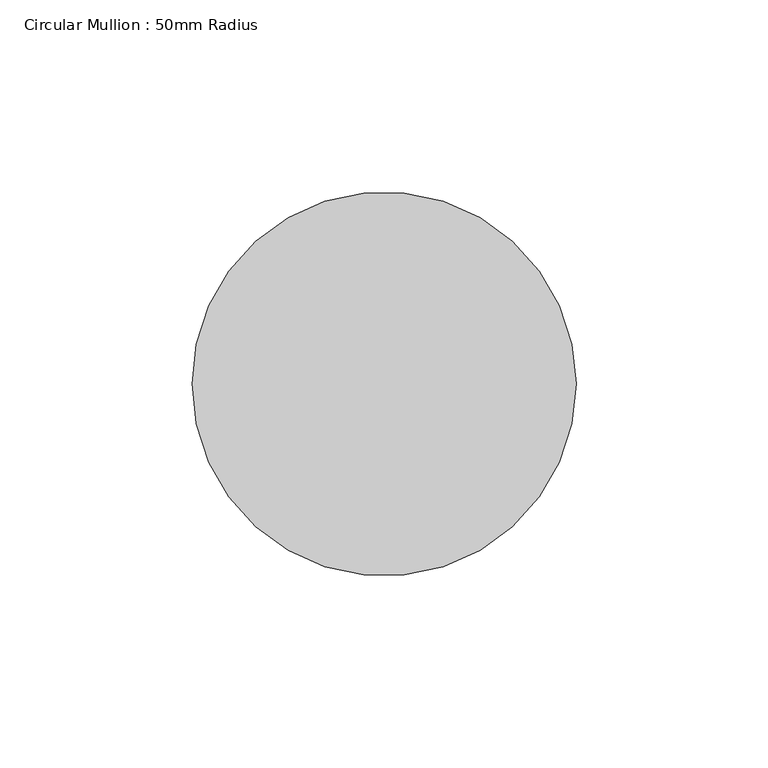
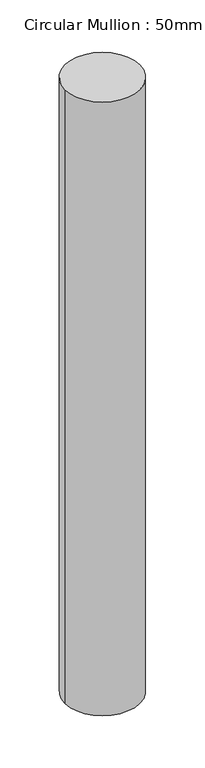
"""IFC4 building model written with IfcOpenShell, lengths in millimetres: member geometry, Circular Mullion : 50mm Radius."""

from ifc_helpers import new_model, si_unit, point, frame, frame_2d, origin, place, context, project, spatial, circle_curve, trimmed, segment, composite_curve, outline, extrude, source, transform, mapped, element, save


def circular_mullion_50mm_radius_89187424(model_context):
    return source(origin(), model_context, "Body", "SweptSolid", [
        extrude(outline(composite_curve([segment(trimmed(circle_curve(frame_2d((-50.0, 0.0)), 50.0), [point((0.0, 0.0))], [point((-100.0, 0.0))], False, "CARTESIAN"), True, "CONTINUOUS"), segment(trimmed(circle_curve(frame_2d((-50.0, 0.0)), 50.0), [point((-100.0, 0.0))], [point((0.0, 0.0))], False, "CARTESIAN"), True, "CONTINUOUS")], self_intersect=False)), frame((0.0, 0.0, -865.2655587), z_axis=(0.0, 0.0, 1.0), x_axis=(1.0, 0.0, 0.0)), (0.0, 0.0, 1.0), 865.2655587),
    ])


if __name__ == "__main__":
    model = new_model("IFC4")
    model_context = context("Model", 3, world=origin())
    ifc_project = project(units=[si_unit("LENGTHUNIT", "METRE", prefix="MILLI")], contexts=[model_context])
    site = spatial("IfcSite", under=ifc_project)
    building = spatial("IfcBuilding", under=site)
    placement = place(None, origin())
    circular_mullion_50mm_radius_shape = circular_mullion_50mm_radius_89187424(model_context)
    element("IfcMember", 1, ObjectType="Circular Mullion : 50mm Radius", at=placement, inside=building, context=model_context, shape_type="MappedRepresentation", body=[
        mapped(circular_mullion_50mm_radius_shape, transform((0.0, 0.0, 0.0), x_axis=(1.0, 0.0, 0.0), y_axis=(0.0, 1.0, 0.0), z_axis=(0.0, 0.0, 1.0))),
    ])
    save(model, "model.ifc")

# Revit data of these elements
# Type "Circular Mullion : 50mm Radius"
#   built-in parameter 1007350 = 0.164042 (stored number, unit not read)
# Element 1 (IfcMember, "Circular Mullion : 50mm Radius")
#   Materials on its faces: "Aluminium"
# Materials
#   "Aluminium": class "Metal", colour RGB 247 247 247, transparency 0, Description = "Aluminium 6061", Cost = 0
